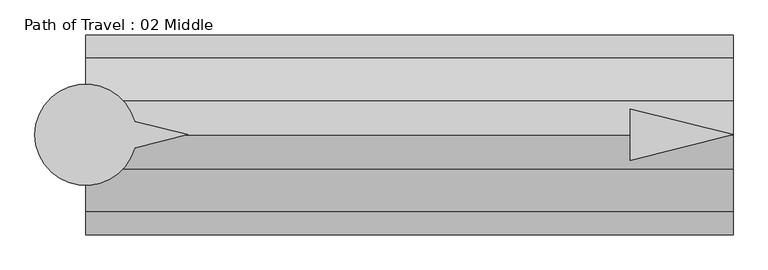
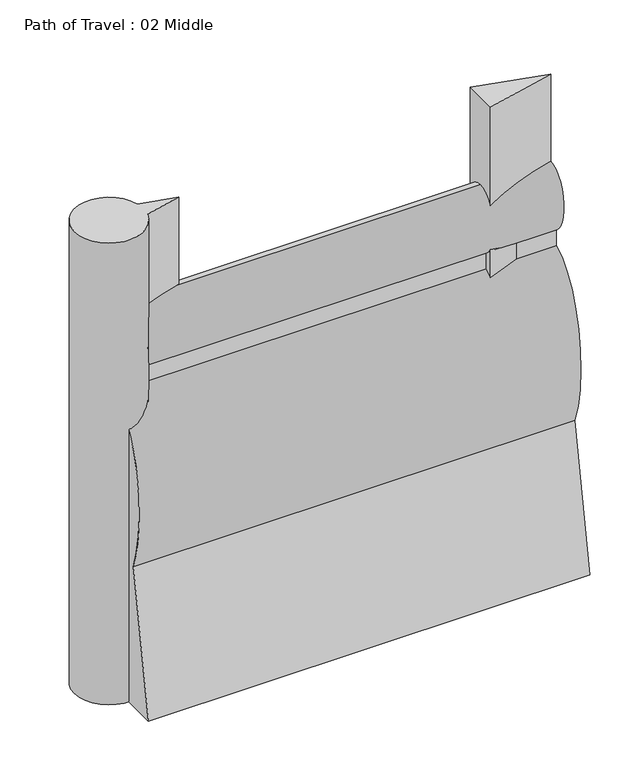
"""IFC4 building model written with IfcOpenShell, lengths in millimetres: proxy geometry, Path of Travel : 02 Middle."""

from ifc_helpers import new_model, si_unit, point, frame, frame_2d, origin, origin_with_axes, place, context, project, spatial, polyline, circle_curve, ellipse_curve, trimmed, segment, composite_curve, outline, extrude, source, transform, mapped, element, save
from ifc_brep_helpers import plane_surface, extruded_surface, advanced_brep


def path_of_travel_02_middle_3647c35c(model_context):
    return source(origin(), model_context, "Body", "SolidModel", [
        advanced_brep(
        [(227.5554837, 0.0, 1727.2), (227.5554837, 42.9018657, 1436.6534209), (227.5554837, 42.9018657, 1363.4763406), (227.5554837, 184.1186263, 643.4144547), (227.5554837, 297.5699544, 0.0), (227.5554837, 145.6574193, 0.0), (227.5554837, 0.0, 584.2), (227.5554837, -145.6574193, 0.0), (227.5554837, -297.5699544, 0.0), (227.5554837, -184.1186263, 643.4144547), (227.5554837, -42.9018657, 1363.4763406), (227.5554837, -42.9018657, 1436.6534209), (2152.1530954, 0.0, 1727.2), (2152.1530954, -42.9018657, 1436.6534209), (2152.1530954, -42.9018657, 1363.4763406), (2152.1530954, -184.1186263, 643.4144547), (2152.1530954, -297.5699544, 0.0), (2152.1530954, -145.6574193, 0.0), (2152.1530954, 0.0, 584.2), (2152.1530954, 145.6574193, 0.0), (2152.1530954, 297.5699544, 0.0), (2152.1530954, 184.1186263, 643.4144547), (2152.1530954, 42.9018657, 1363.4763406), (2152.1530954, 42.9018657, 1436.6534209)],
        [
            (0, 1, ellipse_curve(frame((227.5554837, 0.0, 1574.8), z_axis=(-1.0, 0.0, 0.0), x_axis=(0.0, 0.0, 1.0)), 152.4, 101.6)),
            (1, 2),
            (2, 3, ellipse_curve(frame((227.5554837, 0.0, 914.4), z_axis=(-1.0, 0.0, 0.0), x_axis=(0.0, 0.0, -1.0)), 457.2, 228.6)),
            (3, 4),
            (4, 5),
            (5, 6),
            (6, 7),
            (7, 8),
            (8, 9),
            (9, 10, ellipse_curve(frame((227.5554837, 0.0, 914.4), z_axis=(-1.0, 0.0, 0.0), x_axis=(0.0, 0.0, -1.0)), 457.2, 228.6)),
            (10, 11),
            (11, 0, ellipse_curve(frame((227.5554837, 0.0, 1574.8), z_axis=(-1.0, 0.0, 0.0), x_axis=(0.0, 0.0, 1.0)), 152.4, 101.6)),
            (12, 13, ellipse_curve(frame((2152.1530954, 0.0, 1574.8), z_axis=(1.0, 0.0, 0.0), x_axis=(0.0, 0.0, 1.0)), 152.4, 101.6)),
            (13, 14),
            (14, 15, ellipse_curve(frame((2152.1530954, 0.0, 914.4), z_axis=(1.0, 0.0, 0.0), x_axis=(0.0, 0.0, -1.0)), 457.2, 228.6)),
            (15, 16),
            (16, 17),
            (17, 18),
            (18, 19),
            (19, 20),
            (20, 21),
            (21, 22, ellipse_curve(frame((2152.1530954, 0.0, 914.4), z_axis=(1.0, 0.0, 0.0), x_axis=(0.0, 0.0, -1.0)), 457.2, 228.6)),
            (22, 23),
            (23, 12, ellipse_curve(frame((2152.1530954, 0.0, 1574.8), z_axis=(1.0, 0.0, 0.0), x_axis=(0.0, 0.0, 1.0)), 152.4, 101.6)),
            (0, 12),
            (23, 1),
            (22, 2),
            (21, 3),
            (20, 4),
            (19, 5),
            (18, 6),
            (17, 7),
            (16, 8),
            (15, 9),
            (14, 10),
            (13, 11),
        ],
        [
            plane_surface(frame((227.5554837, 0.0, 0.0), z_axis=(-1.0, 0.0, 0.0), x_axis=(0.0, 0.0, 1.0))),
            plane_surface(frame((2152.1530954, 0.0, 0.0), z_axis=(1.0, 0.0, 0.0), x_axis=(0.0, 0.0, 1.0))),
            extruded_surface(trimmed(ellipse_curve(frame((2152.1530954, 0.0, 1574.8), z_axis=(-1.0, 0.0, 0.0), x_axis=(0.0, 0.0, 1.0)), 152.4, 101.6), [point((2152.1530954, 0.0, 1727.2))], [point((2152.1530954, 42.9018657, 1436.6534209))], True, "CARTESIAN"), (-1924.5976117, 0.0, 0.0), 1924.5976117),
            plane_surface(frame((227.5554837, 42.9018657, 1436.6534209), z_axis=(0.0, 1.0, 0.0), x_axis=(1.0, 0.0, 0.0))),
            extruded_surface(trimmed(ellipse_curve(frame((2152.1530954, 0.0, 914.4), z_axis=(-1.0, 0.0, 0.0), x_axis=(0.0, 0.0, -1.0)), 457.2, 228.6), [point((2152.1530954, 42.9018657, 1363.4763406))], [point((2152.1530954, 184.1186263, 643.4144547))], True, "CARTESIAN"), (-1924.5976117, 0.0, 0.0), 1924.5976117),
            plane_surface(frame((227.5554837, 184.1186263, 643.4144547), z_axis=(0.0, 0.9848077530122078, 0.1736481776669322), x_axis=(1.0, 0.0, 0.0))),
            plane_surface(frame((227.5554837, 297.5699544, 0.0), z_axis=(0.0, 0.0, -1.0), x_axis=(1.0, 0.0, 0.0))),
            plane_surface(frame((227.5554837, 145.6574193, 0.0), z_axis=(0.0, -0.9702957262760199, -0.2419218955995739), x_axis=(1.0, 0.0, 0.0))),
            plane_surface(frame((227.5554837, 0.0, 584.2), z_axis=(0.0, 0.9702957262759961, -0.24192189559966923), x_axis=(1.0, 0.0, 0.0))),
            plane_surface(frame((227.5554837, -145.6574193, 0.0), z_axis=(0.0, 0.0, -1.0), x_axis=(1.0, 0.0, 0.0))),
            plane_surface(frame((227.5554837, -297.5699544, 0.0), z_axis=(0.0, -0.984807753012208, 0.17364817766693066), x_axis=(1.0, 0.0, 0.0))),
            extruded_surface(trimmed(ellipse_curve(frame((2152.1530954, 0.0, 914.4), z_axis=(-1.0, 0.0, 0.0), x_axis=(0.0, 0.0, -1.0)), 457.2, 228.6), [point((2152.1530954, -184.1186263, 643.4144547))], [point((2152.1530954, -42.9018657, 1363.4763406))], True, "CARTESIAN"), (-1924.5976117, 0.0, 0.0), 1924.5976117),
            plane_surface(frame((227.5554837, -42.9018657, 1363.4763406), z_axis=(0.0, -1.0, 0.0), x_axis=(1.0, 0.0, 0.0))),
            extruded_surface(trimmed(ellipse_curve(frame((2152.1530954, 0.0, 1574.8), z_axis=(-1.0, 0.0, 0.0), x_axis=(0.0, 0.0, 1.0)), 152.4, 101.6), [point((2152.1530954, -42.9018657, 1436.6534209))], [point((2152.1530954, 0.0, 1727.2))], True, "CARTESIAN"), (-1924.5976117, 0.0, 0.0), 1924.5976117),
        ],
        [
            (0, [[1, 2, 3, 4, 5, 6, 7, 8, 9, 10, 11, 12]]),
            (1, [[13, 14, 15, 16, 17, 18, 19, 20, 21, 22, 23, 24]]),
            (2, [[-1, 25, -24, 26]]),
            (3, [[-2, -26, -23, 27]]),
            (4, [[-3, -27, -22, 28]]),
            (5, [[-4, -28, -21, 29]]),
            (6, [[-5, -29, -20, 30]]),
            (7, [[-6, -30, -19, 31]]),
            (8, [[-7, -31, -18, 32]]),
            (9, [[-8, -32, -17, 33]]),
            (10, [[-9, -33, -16, 34]]),
            (11, [[-10, -34, -15, 35]]),
            (12, [[-11, -35, -14, 36]]),
            (13, [[-12, -36, -13, -25]]),
        ],
    ),
        extrude(outline(polyline([(1846.1479489, 76.2006338), (2152.1530954, 0.0), (1846.1479489, -76.2006338), (1846.1479489, 76.2006338)])), origin_with_axes(), (0.0, 0.0, 1.0), 2129.5973753),
        extrude(outline(composite_curve([segment(polyline([(372.7837828, 39.4440225), (531.182385, 0.0), (372.7837828, -39.4440225)]), True, "CONTINUOUS"), segment(trimmed(circle_curve(frame_2d((227.2200886, 0.0)), 150.8131956), [point((372.7837828, -39.4440225))], [point((372.7837828, 39.4440225))], False, "CARTESIAN"), True, "CONTINUOUS")], self_intersect=False)), origin_with_axes(), (0.0, 0.0, 1.0), 2129.5973753),
    ])


if __name__ == "__main__":
    model = new_model("IFC4")
    model_context = context("Model", 3, world=origin())
    ifc_project = project(units=[si_unit("LENGTHUNIT", "METRE", prefix="MILLI")], contexts=[model_context])
    site = spatial("IfcSite", under=ifc_project)
    building = spatial("IfcBuilding", under=site)
    placement = place(None, origin())
    path_of_travel_02_middle_shape = path_of_travel_02_middle_3647c35c(model_context)
    element("IfcBuildingElementProxy", 1, Name="Path of Travel : 02 Middle", ObjectType="Path of Travel : 02 Middle", at=placement, inside=building, context=model_context, shape_type="MappedRepresentation", body=[
        mapped(path_of_travel_02_middle_shape, transform((0.0, 0.0, 0.0), x_axis=(1.0, 0.0, 0.0), y_axis=(0.0, 1.0, 0.0), z_axis=(0.0, 0.0, 1.0))),
    ])
    save(model, "model.ifc")

# Revit data of these elements
# Type "Path of Travel : 02 Middle"
#   Path of Egress [instance default] = 4' - 0"
#   built-in parameter 1001306 [instance default] = 4 (stored number, unit not read)
#   Dot at Start = no
#   Arrow in Middle = yes
#   Arrow at End = no
#   Egress Path = none
# Element 1 (IfcBuildingElementProxy, "Path of Travel : 02 Middle")
#   Path of Egress = 6' - 3.77156"
#   built-in parameter 1001306 = 6.3143 (stored number, unit not read)
#   Materials on its faces: "Egress Path Solid", "solid"
# Materials
#   "Egress Path Solid": class "Unassigned", colour RGB 255 128 64, transparency 0.75, Comments = "Rendering appearance not upgraded "
#   "solid": class "Generic", colour RGB 120 120 120, transparency 0, Cost = 0
